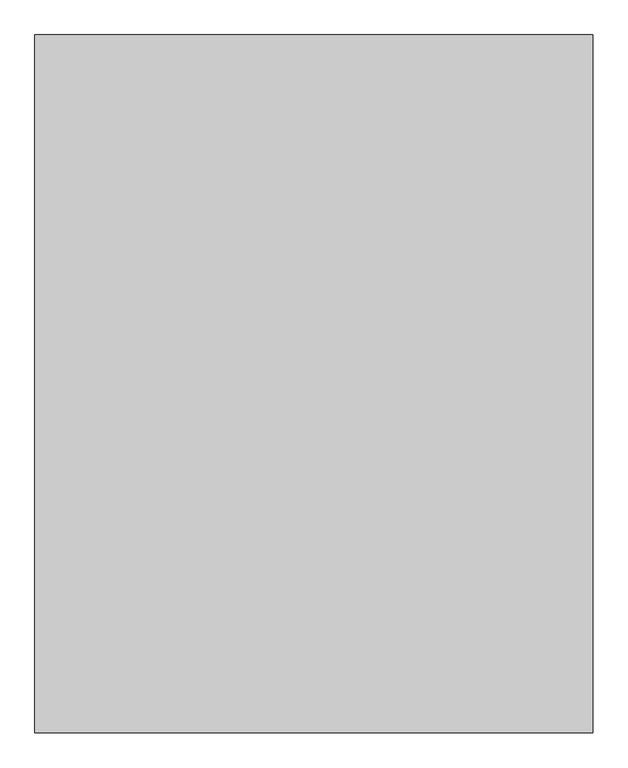
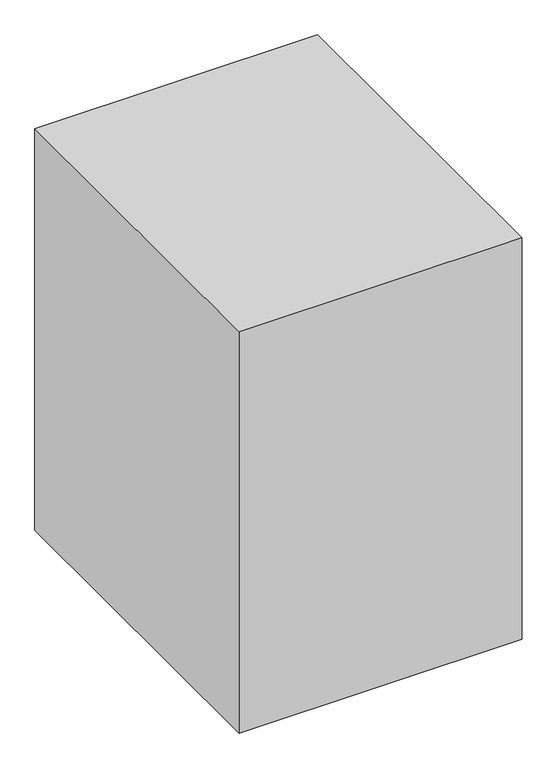
"""IFC4 building model written with IfcOpenShell, lengths in millimetres: proxy geometry, Space Planning Box_hec : Space Planning Box_hec."""

from ifc_helpers import new_model, si_unit, origin, origin_with_axes, place, context, project, spatial, polyline, outline, extrude, source, transform, mapped, element, save


def generic_models_5b7b272c(model_context):
    return source(origin(), model_context, "Body", "SweptSolid", [
        extrude(outline(polyline([(2000.0, 2500.0), (2000.0, -2500.0), (-2000.0, -2500.0), (-2000.0, 2500.0), (2000.0, 2500.0)])), origin_with_axes(), (0.0, 0.0, 1.0), 6000.0),
    ])


if __name__ == "__main__":
    model = new_model("IFC4")
    model_context = context("Model", 3, world=origin())
    ifc_project = project(units=[si_unit("LENGTHUNIT", "METRE", prefix="MILLI")], contexts=[model_context])
    site = spatial("IfcSite", under=ifc_project)
    building = spatial("IfcBuilding", under=site)
    placement = place(None, origin())
    generic_models_shape = generic_models_5b7b272c(model_context)
    element("IfcBuildingElementProxy", 1, Name="Space Planning Box_hec : Space Planning Box_hec", ObjectType="Space Planning Box_hec : Space Planning Box_hec", at=placement, inside=building, context=model_context, shape_type="MappedRepresentation", body=[
        mapped(generic_models_shape, transform((0.0, 0.0, 0.0), x_axis=(1.0, 0.0, 0.0), y_axis=(0.0, 1.0, 0.0), z_axis=(0.0, 0.0, 1.0))),
    ])
    save(model, "model.ifc")

# Revit data of these elements
# Type "Space Planning Box_hec : Space Planning Box_hec"
#   Type Comments = "..."
#   Room Name [instance default] = "?"
#   Interior Finish [instance default] = ""
#   Exterior Finish [instance default] = ""
#   Department [instance default] = ""
#   Assembly Code = "..."
#   Width [instance default] = 1524 mm
#   Program Area [instance default] = 0.00 m²
#   Length [instance default] = 1524 mm
#   Height [instance default] = 1524 mm
#   Area [instance default] = 2.32258 m²
#   Fill Color [instance default] = Cyan
#   Default Elevation = 0
# Element 1 (IfcBuildingElementProxy, "Space Planning Box_hec : Space Planning Box_hec")
#   Room Name = "Toilet (M)"
#   Interior Finish = "IF5"
#   Exterior Finish = "EF1"
#   Department = "AR"
#   Width = 4000 mm
#   Program Area = 72.00 m²
#   Length = 5000 mm
#   Height = 6000 mm
#   Area = 20.00 m²
#   Fill Color = Lavender
#   Materials on its faces: "Lavender"
# Materials
#   "Cyan": class "Generic", colour RGB 0 255 255, transparency 0.2, Cost = 0
#   "Lavender": class "Generic", colour RGB 186 85 211, transparency 0.2, Cost = 0
